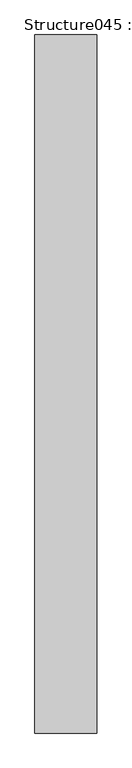
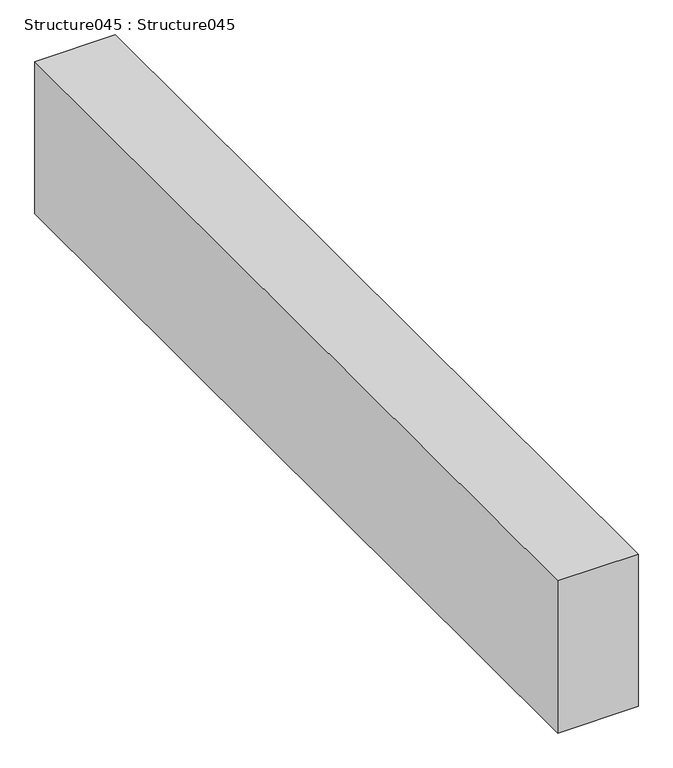
"""IFC4 building model written with IfcOpenShell, lengths in millimetres: proxy geometry, Structure045 : Structure045."""

from ifc_helpers import new_model, si_unit, frame, origin, place, context, project, spatial, polyline, outline, extrude, source, transform, mapped, element, save


def structure045_structure045_ae569b77(model_context):
    return source(origin(), model_context, "Body", "SweptSolid", [
        extrude(outline(polyline([(-2567.3737014, -1052.8906574), (-2745.1737014, -1052.8906574), (-2745.1737014, 947.1093426), (-2567.3737014, 947.1093426), (-2567.3737014, -1052.8906574)])), frame((0.0, 0.0, 39757.096), z_axis=(0.0, 0.0, 1.0), x_axis=(1.0, 0.0, 0.0)), (0.0, 0.0, 1.0), 355.6),
    ])


if __name__ == "__main__":
    model = new_model("IFC4")
    model_context = context("Model", 3, world=origin())
    ifc_project = project(units=[si_unit("LENGTHUNIT", "METRE", prefix="MILLI")], contexts=[model_context])
    site = spatial("IfcSite", under=ifc_project)
    building = spatial("IfcBuilding", under=site)
    placement = place(None, origin())
    structure045_structure045_shape = structure045_structure045_ae569b77(model_context)
    element("IfcBuildingElementProxy", 1, Name="Structure045 : Structure045", ObjectType="Structure045 : Structure045", at=placement, inside=building, context=model_context, shape_type="MappedRepresentation", body=[
        mapped(structure045_structure045_shape, transform((0.0, 0.0, 0.0), x_axis=(1.0, 0.0, 0.0), y_axis=(0.0, 1.0, 0.0), z_axis=(0.0, 0.0, 1.0))),
    ])
    save(model, "model.ifc")

# Revit data of these elements
# Type "Structure045 : Structure045"
#   NameOverride = "Structure045"
# Element 1 (IfcBuildingElementProxy, "Structure045 : Structure045")
#   Materials on its faces: "STRUCTURAL MEMBER (SEE DWGS)"
# Materials
#   "STRUCTURAL MEMBER (SEE DWGS)": class "Unassigned", colour RGB 214 178 158, transparency 0, Cost = 0
